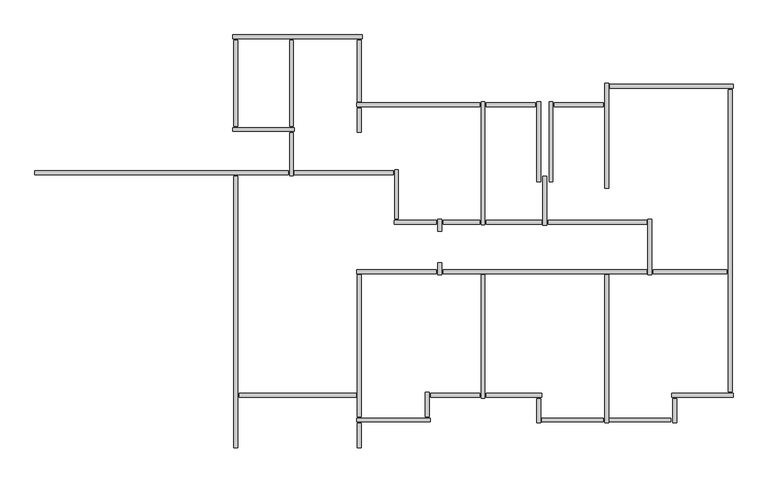
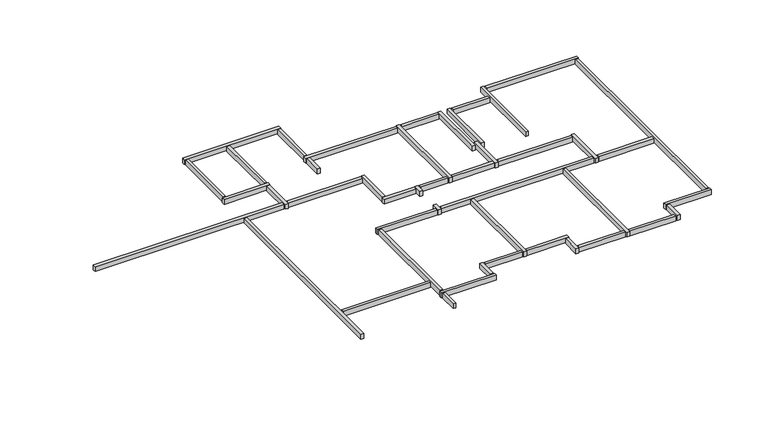
"""IFC4 building model written with IfcOpenShell, lengths in millimetres: beam geometry, Graute viga de respaldo20 : Graute viga de respaldo."""

from ifc_helpers import new_model, si_unit, frame, origin, place, context, project, spatial, polyline, outline, extrude, source, transform, mapped, element, save


def beam_fe787a5c(model_context):
    return source(origin(), model_context, "Body", "SweptSolid", [
        extrude(outline(polyline([(-54994.9587292, 57408.4278788), (-54994.9587292, 57502.4278788), (-53804.9587292, 57502.4278788), (-53804.9587292, 57408.4278788), (-54994.9587292, 57408.4278788)])), frame((0.0, 0.0, 17632.9999999), z_axis=(0.0, 0.0, 1.0), x_axis=(1.0, 0.0, 0.0)), (0.0, 0.0, 1.0), 167.0),
        extrude(outline(polyline([(-56644.9587292, 57408.4278788), (-56644.9587292, 57502.4278788), (-55454.9587292, 57502.4278788), (-55454.9587292, 57408.4278788), (-56644.9587292, 57408.4278788)])), frame((0.0, 0.0, 17632.9999999), z_axis=(0.0, 0.0, 1.0), x_axis=(1.0, 0.0, 0.0)), (0.0, 0.0, 1.0), 167.0),
        extrude(outline(polyline([(-52594.9587292, 53358.4278788), (-52594.9587292, 53452.4278788), (-50804.9587292, 53452.4278788), (-50804.9587292, 53358.4278788), (-52594.9587292, 53358.4278788)])), frame((0.0, 0.0, 17632.9999999), z_axis=(0.0, 0.0, 1.0), x_axis=(1.0, 0.0, 0.0)), (0.0, 0.0, 1.0), 167.0),
        extrude(outline(polyline([(-57994.9587292, 50358.4278788), (-57994.9587292, 50452.4278788), (-56804.9587292, 50452.4278788), (-56804.9587292, 50358.4278788), (-57994.9587292, 50358.4278788)])), frame((0.0, 0.0, 17632.9999999), z_axis=(0.0, 0.0, 1.0), x_axis=(1.0, 0.0, 0.0)), (0.0, 0.0, 1.0), 167.0),
        extrude(outline(polyline([(-58121.9587292, 50475.4278788), (-58027.9587292, 50475.4278788), (-58027.9587292, 49885.4278788), (-58121.9587292, 49885.4278788), (-58121.9587292, 50475.4278788)])), frame((0.0, 0.0, 17632.9999999), z_axis=(0.0, 0.0, 1.0), x_axis=(1.0, 0.0, 0.0)), (0.0, 0.0, 1.0), 167.0),
        extrude(outline(polyline([(-59794.9587292, 49758.4278788), (-59794.9587292, 49852.4278788), (-58004.9587292, 49852.4278788), (-58004.9587292, 49758.4278788), (-59794.9587292, 49758.4278788)])), frame((0.0, 0.0, 17632.9999999), z_axis=(0.0, 0.0, 1.0), x_axis=(1.0, 0.0, 0.0)), (0.0, 0.0, 1.0), 167.0),
        extrude(outline(polyline([(-57727.9587292, 53335.4278788), (-57821.9587292, 53335.4278788), (-57821.9587292, 53625.4278788), (-57727.9587292, 53625.4278788), (-57727.9587292, 53335.4278788)])), frame((0.0, 0.0, 17632.9999999), z_axis=(0.0, 0.0, 1.0), x_axis=(1.0, 0.0, 0.0)), (0.0, 0.0, 1.0), 167.0),
        extrude(outline(polyline([(-55144.9587292, 54558.4278788), (-55144.9587292, 54652.4278788), (-52754.9587292, 54652.4278788), (-52754.9587292, 54558.4278788), (-55144.9587292, 54558.4278788)])), frame((0.0, 0.0, 17632.9999999), z_axis=(0.0, 0.0, 1.0), x_axis=(1.0, 0.0, 0.0)), (0.0, 0.0, 1.0), 167.0),
        extrude(outline(polyline([(-56644.9587292, 54558.4278788), (-56644.9587292, 54652.4278788), (-55304.9587292, 54652.4278788), (-55304.9587292, 54558.4278788), (-56644.9587292, 54558.4278788)])), frame((0.0, 0.0, 17632.9999999), z_axis=(0.0, 0.0, 1.0), x_axis=(1.0, 0.0, 0.0)), (0.0, 0.0, 1.0), 167.0),
        extrude(outline(polyline([(-57694.9587292, 54558.4278788), (-57694.9587292, 54652.4278788), (-56804.9587292, 54652.4278788), (-56804.9587292, 54558.4278788), (-57694.9587292, 54558.4278788)])), frame((0.0, 0.0, 17632.9999999), z_axis=(0.0, 0.0, 1.0), x_axis=(1.0, 0.0, 0.0)), (0.0, 0.0, 1.0), 167.0),
        extrude(outline(polyline([(-57727.9587292, 54385.4278788), (-57821.9587292, 54385.4278788), (-57821.9587292, 54675.4278788), (-57727.9587292, 54675.4278788), (-57727.9587292, 54385.4278788)])), frame((0.0, 0.0, 17632.9999999), z_axis=(0.0, 0.0, 1.0), x_axis=(1.0, 0.0, 0.0)), (0.0, 0.0, 1.0), 167.0),
        extrude(outline(polyline([(-58884.9587292, 54558.4278788), (-58884.9587292, 54652.4278788), (-57854.9587292, 54652.4278788), (-57854.9587292, 54558.4278788), (-58884.9587292, 54558.4278788)])), frame((0.0, 0.0, 17632.9999999), z_axis=(0.0, 0.0, 1.0), x_axis=(1.0, 0.0, 0.0)), (0.0, 0.0, 1.0), 167.0),
        extrude(outline(polyline([(-58871.9587292, 55875.4278788), (-58777.9587292, 55875.4278788), (-58777.9587292, 54685.4278788), (-58871.9587292, 54685.4278788), (-58871.9587292, 55875.4278788)])), frame((0.0, 0.0, 17632.9999999), z_axis=(0.0, 0.0, 1.0), x_axis=(1.0, 0.0, 0.0)), (0.0, 0.0, 1.0), 167.0),
        extrude(outline(polyline([(-61304.9587292, 55758.4278788), (-61304.9587292, 55852.4278788), (-58904.9587292, 55852.4278788), (-58904.9587292, 55758.4278788), (-61304.9587292, 55758.4278788)])), frame((0.0, 0.0, 17632.9999999), z_axis=(0.0, 0.0, 1.0), x_axis=(1.0, 0.0, 0.0)), (0.0, 0.0, 1.0), 167.0),
        extrude(outline(polyline([(-56677.9587292, 54540.4278788), (-56771.9587292, 54540.4278788), (-56771.9587292, 57525.4278788), (-56677.9587292, 57525.4278788), (-56677.9587292, 54540.4278788)])), frame((0.0, 0.0, 17632.9999999), z_axis=(0.0, 0.0, 1.0), x_axis=(1.0, 0.0, 0.0)), (0.0, 0.0, 1.0), 167.0),
        extrude(outline(polyline([(-59794.9587292, 57408.4278788), (-59794.9587292, 57502.4278788), (-56804.9587292, 57502.4278788), (-56804.9587292, 57408.4278788), (-59794.9587292, 57408.4278788)])), frame((0.0, 0.0, 17632.9999999), z_axis=(0.0, 0.0, 1.0), x_axis=(1.0, 0.0, 0.0)), (0.0, 0.0, 1.0), 167.0),
        extrude(outline(polyline([(-59677.9587292, 56785.4278788), (-59771.9587292, 56785.4278788), (-59771.9587292, 57375.4278788), (-59677.9587292, 57375.4278788), (-59677.9587292, 56785.4278788)])), frame((0.0, 0.0, 17632.9999999), z_axis=(0.0, 0.0, 1.0), x_axis=(1.0, 0.0, 0.0)), (0.0, 0.0, 1.0), 167.0),
        extrude(outline(polyline([(-59771.9587292, 59025.4278788), (-59677.9587292, 59025.4278788), (-59677.9587292, 57535.4278788), (-59771.9587292, 57535.4278788), (-59771.9587292, 59025.4278788)])), frame((0.0, 0.0, 17632.9999999), z_axis=(0.0, 0.0, 1.0), x_axis=(1.0, 0.0, 0.0)), (0.0, 0.0, 1.0), 167.0),
        extrude(outline(polyline([(-62771.9587292, 59025.4278788), (-62677.9587292, 59025.4278788), (-62677.9587292, 56935.4278788), (-62771.9587292, 56935.4278788), (-62771.9587292, 59025.4278788)])), frame((0.0, 0.0, 17632.9999999), z_axis=(0.0, 0.0, 1.0), x_axis=(1.0, 0.0, 0.0)), (0.0, 0.0, 1.0), 167.0),
        extrude(outline(polyline([(-61421.9587292, 59025.4278788), (-61327.9587292, 59025.4278788), (-61327.9587292, 56935.4278788), (-61421.9587292, 56935.4278788), (-61421.9587292, 59025.4278788)])), frame((0.0, 0.0, 17632.9999999), z_axis=(0.0, 0.0, 1.0), x_axis=(1.0, 0.0, 0.0)), (0.0, 0.0, 1.0), 167.0),
        extrude(outline(polyline([(-61327.9587292, 55735.4278788), (-61421.9587292, 55735.4278788), (-61421.9587292, 56775.4278788), (-61327.9587292, 56775.4278788), (-61327.9587292, 55735.4278788)])), frame((0.0, 0.0, 17632.9999999), z_axis=(0.0, 0.0, 1.0), x_axis=(1.0, 0.0, 0.0)), (0.0, 0.0, 1.0), 167.0),
        extrude(outline(polyline([(-62644.9587292, 50358.4278788), (-62644.9587292, 50452.4278788), (-59804.9587292, 50452.4278788), (-59804.9587292, 50358.4278788), (-62644.9587292, 50358.4278788)])), frame((0.0, 0.0, 17632.9999999), z_axis=(0.0, 0.0, 1.0), x_axis=(1.0, 0.0, 0.0)), (0.0, 0.0, 1.0), 167.0),
        extrude(outline(polyline([(-59771.9587292, 53325.4278788), (-59677.9587292, 53325.4278788), (-59677.9587292, 49885.4278788), (-59771.9587292, 49885.4278788), (-59771.9587292, 53325.4278788)])), frame((0.0, 0.0, 17632.9999999), z_axis=(0.0, 0.0, 1.0), x_axis=(1.0, 0.0, 0.0)), (0.0, 0.0, 1.0), 167.0),
        extrude(outline(polyline([(-59794.9587292, 53358.4278788), (-59794.9587292, 53452.4278788), (-57854.9587292, 53452.4278788), (-57854.9587292, 53358.4278788), (-59794.9587292, 53358.4278788)])), frame((0.0, 0.0, 17632.9999999), z_axis=(0.0, 0.0, 1.0), x_axis=(1.0, 0.0, 0.0)), (0.0, 0.0, 1.0), 167.0),
        extrude(outline(polyline([(-57694.9587292, 53358.4278788), (-57694.9587292, 53452.4278788), (-52754.9587292, 53452.4278788), (-52754.9587292, 53358.4278788), (-57694.9587292, 53358.4278788)])), frame((0.0, 0.0, 17632.9999999), z_axis=(0.0, 0.0, 1.0), x_axis=(1.0, 0.0, 0.0)), (0.0, 0.0, 1.0), 167.0),
        extrude(outline(polyline([(-56677.9587292, 50335.4278788), (-56771.9587292, 50335.4278788), (-56771.9587292, 53325.4278788), (-56677.9587292, 53325.4278788), (-56677.9587292, 50335.4278788)])), frame((0.0, 0.0, 17632.9999999), z_axis=(0.0, 0.0, 1.0), x_axis=(1.0, 0.0, 0.0)), (0.0, 0.0, 1.0), 167.0),
        extrude(outline(polyline([(-55304.9587292, 50452.4278788), (-55304.9587292, 50358.4278788), (-56644.9587292, 50358.4278788), (-56644.9587292, 50452.4278788), (-55304.9587292, 50452.4278788)])), frame((0.0, 0.0, 17632.9999999), z_axis=(0.0, 0.0, 1.0), x_axis=(1.0, 0.0, 0.0)), (0.0, 0.0, 1.0), 167.0),
        extrude(outline(polyline([(-55327.9587292, 49735.4278788), (-55421.9587292, 49735.4278788), (-55421.9587292, 50325.4278788), (-55327.9587292, 50325.4278788), (-55327.9587292, 49735.4278788)])), frame((0.0, 0.0, 17632.9999999), z_axis=(0.0, 0.0, 1.0), x_axis=(1.0, 0.0, 0.0)), (0.0, 0.0, 1.0), 167.0),
        extrude(outline(polyline([(-55294.9587292, 49758.4278788), (-55294.9587292, 49852.4278788), (-53804.9587292, 49852.4278788), (-53804.9587292, 49758.4278788), (-55294.9587292, 49758.4278788)])), frame((0.0, 0.0, 17632.9999999), z_axis=(0.0, 0.0, 1.0), x_axis=(1.0, 0.0, 0.0)), (0.0, 0.0, 1.0), 167.0),
        extrude(outline(polyline([(-52165.9809043, 49853.4278788), (-52165.9809043, 49758.4278788), (-53654.9587292, 49758.4278788), (-53654.9587292, 49853.4278788), (-52165.9809043, 49853.4278788)])), frame((0.0, 0.0, 17617.1856208), z_axis=(0.0, 0.0, 1.0), x_axis=(1.0, 0.0, 0.0)), (0.0, 0.0, 1.0), 165.0),
        extrude(outline(polyline([(-50771.9587292, 57825.4278788), (-50677.9587292, 57825.4278788), (-50677.9587292, 50485.4278788), (-50771.9587292, 50485.4278788), (-50771.9587292, 57825.4278788)])), frame((0.0, 0.0, 17632.9999999), z_axis=(0.0, 0.0, 1.0), x_axis=(1.0, 0.0, 0.0)), (0.0, 0.0, 1.0), 167.0),
        extrude(outline(polyline([(-52721.9587292, 54675.4278788), (-52627.9587292, 54675.4278788), (-52627.9587292, 53330.0746661), (-52721.9587292, 53330.0746661), (-52721.9587292, 54675.4278788)])), frame((0.0, 0.0, 17632.9999999), z_axis=(0.0, 0.0, 1.0), x_axis=(1.0, 0.0, 0.0)), (0.0, 0.0, 1.0), 167.0),
        extrude(outline(polyline([(-55271.9587292, 55725.4278788), (-55177.9587292, 55725.4278788), (-55177.9587292, 54535.4278788), (-55271.9587292, 54535.4278788), (-55271.9587292, 55725.4278788)])), frame((0.0, 0.0, 17632.9999999), z_axis=(0.0, 0.0, 1.0), x_axis=(1.0, 0.0, 0.0)), (0.0, 0.0, 1.0), 167.0),
        extrude(outline(polyline([(-55121.9587292, 57525.4278788), (-55027.9587292, 57525.4278788), (-55027.9587292, 55585.4278788), (-55121.9587292, 55585.4278788), (-55121.9587292, 57525.4278788)])), frame((0.0, 0.0, 17632.9999999), z_axis=(0.0, 0.0, 1.0), x_axis=(1.0, 0.0, 0.0)), (0.0, 0.0, 1.0), 167.0),
        extrude(outline(polyline([(-55421.9587292, 57525.4278788), (-55327.9587292, 57525.4278788), (-55327.9587292, 55585.4278788), (-55421.9587292, 55585.4278788), (-55421.9587292, 57525.4278788)])), frame((0.0, 0.0, 17632.9999999), z_axis=(0.0, 0.0, 1.0), x_axis=(1.0, 0.0, 0.0)), (0.0, 0.0, 1.0), 167.0),
        extrude(outline(polyline([(-53771.9587292, 57975.4278788), (-53677.9587292, 57975.4278788), (-53677.9587292, 55435.4278788), (-53771.9587292, 55435.4278788), (-53771.9587292, 57975.4278788)])), frame((0.0, 0.0, 17632.9999999), z_axis=(0.0, 0.0, 1.0), x_axis=(1.0, 0.0, 0.0)), (0.0, 0.0, 1.0), 167.0),
        extrude(outline(polyline([(-50654.9587292, 57952.4278788), (-50654.9587292, 57858.4278788), (-53644.9587292, 57858.4278788), (-53644.9587292, 57952.4278788), (-50654.9587292, 57952.4278788)])), frame((0.0, 0.0, 17632.9999999), z_axis=(0.0, 0.0, 1.0), x_axis=(1.0, 0.0, 0.0)), (0.0, 0.0, 1.0), 167.0),
        extrude(outline(polyline([(-52027.9587292, 49735.4278788), (-52121.9587292, 49735.4278788), (-52121.9587292, 50325.4278788), (-52027.9587292, 50325.4278788), (-52027.9587292, 49735.4278788)])), frame((0.0, 0.0, 17632.9999999), z_axis=(0.0, 0.0, 1.0), x_axis=(1.0, 0.0, 0.0)), (0.0, 0.0, 1.0), 167.0),
        extrude(outline(polyline([(-52144.9587292, 50358.4278788), (-52144.9587292, 50452.4278788), (-50654.9587292, 50452.4278788), (-50654.9587292, 50358.4278788), (-52144.9587292, 50358.4278788)])), frame((0.0, 0.0, 17632.9999999), z_axis=(0.0, 0.0, 1.0), x_axis=(1.0, 0.0, 0.0)), (0.0, 0.0, 1.0), 167.0),
        extrude(outline(polyline([(-53677.9587292, 49735.4278788), (-53771.9587292, 49735.4278788), (-53771.9587292, 53325.4278788), (-53677.9587292, 53325.4278788), (-53677.9587292, 49735.4278788)])), frame((0.0, 0.0, 17632.9999999), z_axis=(0.0, 0.0, 1.0), x_axis=(1.0, 0.0, 0.0)), (0.0, 0.0, 1.0), 167.0),
        extrude(outline(polyline([(-59677.9587292, 49135.4278788), (-59771.9587292, 49135.4278788), (-59771.9587292, 49725.4278788), (-59677.9587292, 49725.4278788), (-59677.9587292, 49135.4278788)])), frame((0.0, 0.0, 17632.9999999), z_axis=(0.0, 0.0, 1.0), x_axis=(1.0, 0.0, 0.0)), (0.0, 0.0, 1.0), 167.0),
        extrude(outline(polyline([(-62794.9587292, 56808.4278788), (-62794.9587292, 56902.4278788), (-61304.9587292, 56902.4278788), (-61304.9587292, 56808.4278788), (-62794.9587292, 56808.4278788)])), frame((0.0, 0.0, 17632.9999999), z_axis=(0.0, 0.0, 1.0), x_axis=(1.0, 0.0, 0.0)), (0.0, 0.0, 1.0), 167.0),
        extrude(outline(polyline([(-62794.9587292, 59058.4278788), (-62794.9587292, 59152.4278788), (-59654.9587292, 59152.4278788), (-59654.9587292, 59058.4278788), (-62794.9587292, 59058.4278788)])), frame((0.0, 0.0, 17632.9999999), z_axis=(0.0, 0.0, 1.0), x_axis=(1.0, 0.0, 0.0)), (0.0, 0.0, 1.0), 167.0),
        extrude(outline(polyline([(-67601.7587292, 55758.4278788), (-67601.7587292, 55852.4278788), (-61454.9587292, 55852.4278788), (-61454.9587292, 55758.4278788), (-67601.7587292, 55758.4278788)])), frame((0.0, 0.0, 17632.9999999), z_axis=(0.0, 0.0, 1.0), x_axis=(1.0, 0.0, 0.0)), (0.0, 0.0, 1.0), 167.0),
        extrude(outline(polyline([(-62677.9587292, 49132.8979841), (-62771.9587292, 49132.8979841), (-62771.9587292, 55725.4278788), (-62677.9587292, 55725.4278788), (-62677.9587292, 49132.8979841)])), frame((0.0, 0.0, 17632.9999999), z_axis=(0.0, 0.0, 1.0), x_axis=(1.0, 0.0, 0.0)), (0.0, 0.0, 1.0), 167.0),
    ])


if __name__ == "__main__":
    model = new_model("IFC4")
    model_context = context("Model", 3, world=origin())
    ifc_project = project(units=[si_unit("LENGTHUNIT", "METRE", prefix="MILLI")], contexts=[model_context])
    site = spatial("IfcSite", under=ifc_project)
    building = spatial("IfcBuilding", under=site)
    placement = place(None, origin())
    beam_shape = beam_fe787a5c(model_context)
    element("IfcBeam", 1, ObjectType="Graute viga de respaldo20 : Graute viga de respaldo", at=placement, inside=building, context=model_context, shape_type="MappedRepresentation", body=[
        mapped(beam_shape, transform((0.0, 0.0, 0.0), x_axis=(1.0, 0.0, 0.0), y_axis=(0.0, 1.0, 0.0), z_axis=(0.0, 0.0, 1.0))),
    ])
    save(model, "model.ifc")

# Revit data of these elements
# Element 1 (IfcBeam, "Graute viga de respaldo20 : Graute viga de respaldo")
#   Materials on its faces: "Concreto, Faixa de areia/cimento"
# Materials
#   "Concreto, Faixa de areia/cimento": class "Concreto", colour RGB 127 127 127, transparency 0, Description = "Revestimento de laje de concreto", Cost = 0
